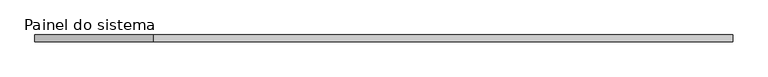
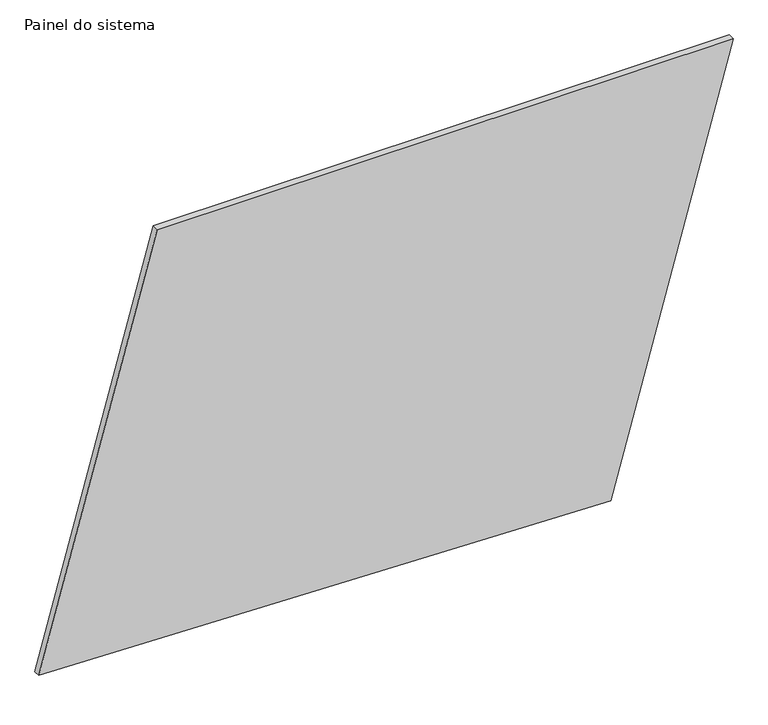
"""IFC4 building model written with IfcOpenShell, lengths in millimetres: plate geometry, Painel do sistema : Envidraçado."""

from ifc_helpers import new_model, si_unit, frame, origin, place, context, project, spatial, polyline, outline, extrude, source, transform, mapped, element, save


def painel_do_sistema_1dea54d0(model_context):
    return source(origin(), model_context, "Body", "SweptSolid", [
        extrude(outline(polyline([(57.4433642, -1288.8045533), (0.0, 833.8436021), (1653.8301049, 1288.8045533), (1653.8301049, -849.6460037), (57.4433642, -1288.8045533)])), frame((0.0, 24.5, 0.0), z_axis=(0.0, 1.0, 0.0), x_axis=(0.0, 0.0, 1.0)), (0.0, 0.0, 1.0), 25.0),
    ])


if __name__ == "__main__":
    model = new_model("IFC4")
    model_context = context("Model", 3, world=origin())
    ifc_project = project(units=[si_unit("LENGTHUNIT", "METRE", prefix="MILLI")], contexts=[model_context])
    site = spatial("IfcSite", under=ifc_project)
    building = spatial("IfcBuilding", under=site)
    placement = place(None, origin())
    painel_do_sistema_shape = painel_do_sistema_1dea54d0(model_context)
    element("IfcPlate", 1, ObjectType="Painel do sistema : Envidraçado", at=placement, inside=building, context=model_context, shape_type="MappedRepresentation", body=[
        mapped(painel_do_sistema_shape, transform((0.0, 0.0, 0.0), x_axis=(1.0, 0.0, 0.0), y_axis=(0.0, 1.0, 0.0), z_axis=(0.0, 0.0, 1.0))),
    ])
    save(model, "model.ifc")

# Revit data of these elements
# Type "Painel do sistema : Envidraçado"
#   Construction Type Id = "GSP4R"
#   Analytic Construction = "Vidraça única Pilkington 1/8 pol"
#   Visual Light Transmittance = 0.9
#   Solar Heat Gain Coefficient = 0.86
#   Heat Transfer Coefficient (U) = 6.7069 W/(m²·K)
# Element 1 (IfcPlate, "Painel do sistema : Envidraçado")
#   Materials on its faces: "Vidro"
# Materials
#   "Vidro": class "Vidro", colour RGB 0 128 192, transparency 0.9, Description = "Vidro de sílica", Cost = 0
